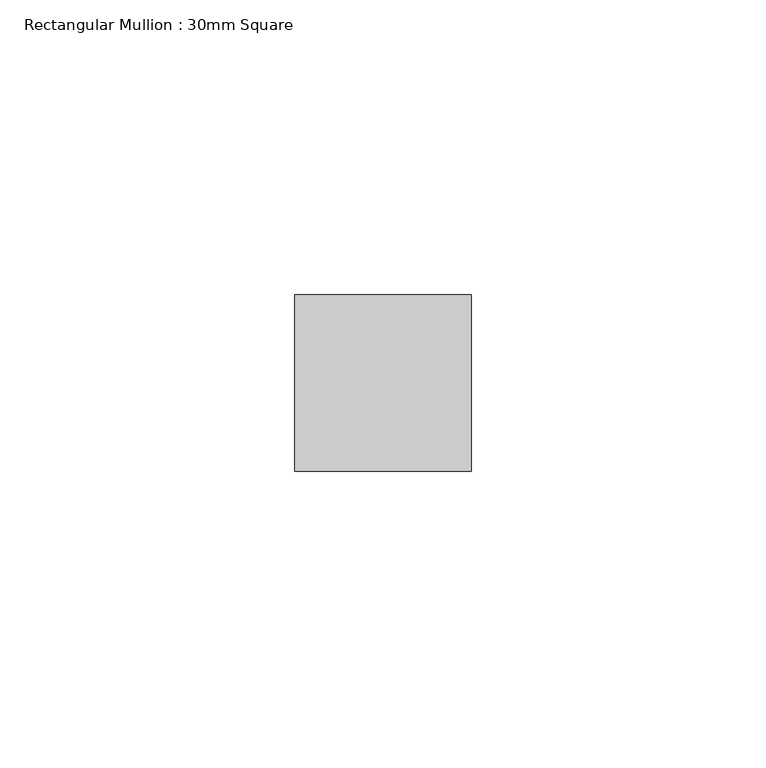
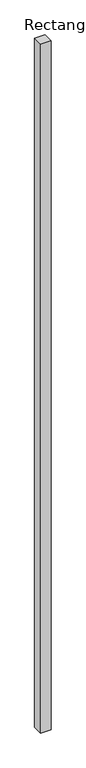
"""IFC4 building model written with IfcOpenShell, lengths in millimetres: member geometry, Rectangular Mullion : 30mm Square."""

import ifcopenshell
import ifcopenshell.guid

model = None  # the IFC model being written
_history = None  # IfcOwnerHistory: only IFC2X3 demands one
_inside = {}  # id of a spatial element -> (the spatial element, [elements in it])
_under = {}  # id of a project, library or spatial element -> (it, [spatial elements below it])
_declared = {}  # id of a project -> (the project, [libraries it declares])
_typed = {}  # id of a type object -> (the type object, [elements of that type])
_made_of = {}  # id of a material, layer set ... -> (it, [elements and type objects made of it])


def new_model(schema):
    """Start an empty IFC model of exactly this schema.

    Asked for "IFC4X3", IfcOpenShell would pick the latest addendum, in which some entities
    have other attributes; the version numbers below select the first issue.
    IFC2X3 requires an IfcOwnerHistory on every rooted entity: one is made here for all.
    """
    global model, _history
    if schema == "IFC4X3":
        model = ifcopenshell.file(schema_version=(4, 3, 0, 0))
    else:
        model = ifcopenshell.file(schema=schema)
    _inside.clear()
    _under.clear()
    _declared.clear()
    _typed.clear()
    _made_of.clear()
    _history = None
    if model.schema == "IFC2X3":
        org = make("IfcOrganization", Name="unknown")
        user = make(
            "IfcPersonAndOrganization",
            ThePerson=make("IfcPerson", FamilyName="unknown"),
            TheOrganization=org,
        )
        app = make(
            "IfcApplication",
            ApplicationDeveloper=org,
            Version="unknown",
            ApplicationFullName="unknown",
            ApplicationIdentifier="unknown",
        )
        _history = make(
            "IfcOwnerHistory",
            OwningUser=user,
            OwningApplication=app,
            ChangeAction="ADDED",
            CreationDate=0,
        )
    return model


def make(cls, **values):
    """One entity of the class cls with the attributes given. An attribute that is None is left unset."""
    return model.create_entity(
        cls, **{name: value for name, value in values.items() if value is not None}
    )


def rooted(cls, **values):
    """An entity with a GlobalId (a new one), such as an element, a storey or a relation."""
    return make(cls, GlobalId=ifcopenshell.guid.new(), OwnerHistory=_history, **values)


def si_unit(unit_type, name, prefix=None):
    """IfcSIUnit, for example si_unit("LENGTHUNIT", "METRE", prefix="MILLI")."""
    return make("IfcSIUnit", UnitType=unit_type, Prefix=prefix, Name=name)


def assignment(units):
    """IfcUnitAssignment: the units of a project."""
    return None if units is None else make("IfcUnitAssignment", Units=units)


def point(xyz):
    """IfcCartesianPoint."""
    return None if xyz is None else make("IfcCartesianPoint", Coordinates=xyz)


def direction(xyz):
    """IfcDirection."""
    return None if xyz is None else make("IfcDirection", DirectionRatios=xyz)


def frame(location, z_axis=None, x_axis=None):
    """IfcAxis2Placement3D, a coordinate frame: its origin and axes. An axis left out is left unset."""
    return make(
        "IfcAxis2Placement3D",
        Location=point(location),
        Axis=direction(z_axis),
        RefDirection=direction(x_axis),
    )


def origin():
    """The frame at (0, 0, 0) with its axes left unset."""
    return frame((0.0, 0.0, 0.0))


def place(relative_to, where):
    """IfcLocalPlacement: puts the frame where relative to a parent placement (None: the world)."""
    return make(
        "IfcLocalPlacement", PlacementRelTo=relative_to, RelativePlacement=where
    )


def context(
    kind, dimensions, precision=None, world=None, true_north=None, identifier=None
):
    """IfcGeometricRepresentationContext, for example the 3D "Model" context."""
    return make(
        "IfcGeometricRepresentationContext",
        ContextIdentifier=identifier,
        ContextType=kind,
        CoordinateSpaceDimension=dimensions,
        Precision=precision,
        WorldCoordinateSystem=world,
        TrueNorth=true_north,
    )


def project(units=None, contexts=None):
    """IfcProject with its units and contexts."""
    return rooted(
        "IfcProject",
        Name="project",
        RepresentationContexts=contexts,
        UnitsInContext=assignment(units),
    )


def spatial(cls, under=None, at=None, **own):
    """A site, building, storey or space (cls), placed at a placement, below another one or the project."""
    s = rooted(cls, ObjectPlacement=at, **own)
    if under is not None:
        _under.setdefault(under.id(), (under, []))[1].append(s)
    return s


def polyline(points):
    """IfcPolyline through the points."""
    return make("IfcPolyline", Points=[point(p) for p in points])


def outline(outer, holes=None, kind="AREA"):
    """IfcArbitraryClosedProfileDef: a profile drawn as a closed curve; with holes, ...WithVoids."""
    if holes is None:
        return make("IfcArbitraryClosedProfileDef", ProfileType=kind, OuterCurve=outer)
    return make(
        "IfcArbitraryProfileDefWithVoids",
        ProfileType=kind,
        OuterCurve=outer,
        InnerCurves=holes,
    )


def extrude(swept, where, along, depth):
    """IfcExtrudedAreaSolid: the profile swept, set in the frame where, extruded along a direction by depth."""
    return make(
        "IfcExtrudedAreaSolid",
        SweptArea=swept,
        Position=where,
        ExtrudedDirection=direction(along),
        Depth=depth,
    )


def shape(context_of_items, identifier, shape_type, items):
    """IfcShapeRepresentation: the items that make up one representation, for example the "Body"."""
    return make(
        "IfcShapeRepresentation",
        ContextOfItems=context_of_items,
        RepresentationIdentifier=identifier,
        RepresentationType=shape_type,
        Items=items,
    )


def source(mapping_origin, context_of_items, identifier, shape_type, items):
    """IfcRepresentationMap: a shape defined once, which mapped items show again and again."""
    return make(
        "IfcRepresentationMap",
        MappingOrigin=mapping_origin,
        MappedRepresentation=shape(context_of_items, identifier, shape_type, items),
    )


def transform(
    local_origin,
    x_axis=None,
    y_axis=None,
    z_axis=None,
    scale=None,
    scale2=None,
    scale3=None,
    uniform=True,
):
    """IfcCartesianTransformationOperator3D, or its non-uniform kind. x_axis, y_axis, z_axis: its Axis1, 2, 3."""
    if uniform:
        return make(
            "IfcCartesianTransformationOperator3D",
            Axis1=direction(x_axis),
            Axis2=direction(y_axis),
            LocalOrigin=point(local_origin),
            Scale=scale,
            Axis3=direction(z_axis),
        )
    return make(
        "IfcCartesianTransformationOperator3DnonUniform",
        Axis1=direction(x_axis),
        Axis2=direction(y_axis),
        LocalOrigin=point(local_origin),
        Scale=scale,
        Axis3=direction(z_axis),
        Scale2=scale2,
        Scale3=scale3,
    )


def mapped(mapping_source, mapping_target):
    """IfcMappedItem: shows the shape of a source again, moved by a transform."""
    return make(
        "IfcMappedItem", MappingSource=mapping_source, MappingTarget=mapping_target
    )


def made_of(thing, what):
    """Note that an element or type object is made of a material, layer set ...; save() writes the relation."""
    if what is not None:
        _made_of.setdefault(what.id(), (what, []))[1].append(thing)
    return thing


def element(
    cls,
    number,
    at=None,
    inside=None,
    cuts=None,
    type_object=None,
    material=None,
    context=None,
    identifier="Body",
    shape_type=None,
    held_by="IfcProductDefinitionShape",
    body=None,
    shapes=None,
    **own,
):
    """One element of the class cls, such as IfcWall. Its Tag is "e" and its number.

    at: its placement. inside: the storey or other place that contains it. cuts: it is an
    opening in that element (IfcRelVoidsElement). A single representation is given by context,
    identifier, shape_type and body (its items); several are given by shapes. held_by: the class
    of the entity that holds the representations. save() writes the other relations.
    """
    e = rooted(cls, Tag="e%d" % number, ObjectPlacement=at, **own)
    if body is not None:
        shapes = [shape(context, identifier, shape_type, body)]
    if shapes is not None:
        e.Representation = make(held_by, Representations=shapes)
    if inside is not None:
        _inside.setdefault(inside.id(), (inside, []))[1].append(e)
    if cuts is not None:
        rooted(
            "IfcRelVoidsElement", RelatingBuildingElement=cuts, RelatedOpeningElement=e
        )
    if type_object is not None:
        _typed.setdefault(type_object.id(), (type_object, []))[1].append(e)
    return made_of(e, material)


def aggregate(whole, parts):
    """IfcRelAggregates: a whole, such as a stair, and the parts it consists of."""
    return rooted("IfcRelAggregates", RelatingObject=whole, RelatedObjects=parts)


def save(model, path):
    """Write the relations noted so far, then the file.

    IfcRelAggregates (storeys below a building ...), IfcRelContainedInSpatialStructure (elements
    in a storey), IfcRelDefinesByType, IfcRelAssociatesMaterial and IfcRelDeclares: one each for
    every whole, place, type object, material and project.
    """
    for whole, parts in _under.values():
        aggregate(whole, parts)
    for where, things in _inside.values():
        rooted(
            "IfcRelContainedInSpatialStructure",
            RelatedElements=things,
            RelatingStructure=where,
        )
    for kind, things in _typed.values():
        rooted("IfcRelDefinesByType", RelatedObjects=things, RelatingType=kind)
    for what, things in _made_of.values():
        rooted("IfcRelAssociatesMaterial", RelatedObjects=things, RelatingMaterial=what)
    for by, libraries in _declared.values():
        rooted("IfcRelDeclares", RelatingContext=by, RelatedDefinitions=libraries)
    model.write(path)


def rectangular_mullion_30mm_square_12e3d361(model_context):
    return source(origin(), model_context, "Body", "SweptSolid", [
        extrude(outline(polyline([(15.0, 15.0), (15.0, -15.0), (-15.0, -15.0), (-15.0, 15.0), (15.0, 15.0)])), frame((0.0, 0.0, -2100.6682892), z_axis=(0.0, 0.0, 1.0), x_axis=(1.0, 0.0, 0.0)), (0.0, 0.0, 1.0), 2100.6682892),
    ])


if __name__ == "__main__":
    model = new_model("IFC4")
    model_context = context("Model", 3, world=origin())
    ifc_project = project(units=[si_unit("LENGTHUNIT", "METRE", prefix="MILLI")], contexts=[model_context])
    site = spatial("IfcSite", under=ifc_project)
    building = spatial("IfcBuilding", under=site)
    placement = place(None, origin())
    rectangular_mullion_30mm_square_shape = rectangular_mullion_30mm_square_12e3d361(model_context)
    element("IfcMember", 1, ObjectType="Rectangular Mullion : 30mm Square", at=placement, inside=building, context=model_context, shape_type="MappedRepresentation", body=[
        mapped(rectangular_mullion_30mm_square_shape, transform((0.0, 0.0, 0.0), x_axis=(1.0, 0.0, 0.0), y_axis=(0.0, 1.0, 0.0), z_axis=(0.0, 0.0, 1.0))),
    ])
    save(model, "model.ifc")

# Revit data of these elements
# Type "Rectangular Mullion : 30mm Square"
#   built-in parameter 1007304 = 0.0984252 (stored number, unit not read)
#   built-in parameter 1007301 = 0.0492126 (stored number, unit not read)
#   built-in parameter 1007300 = 0.0492126 (stored number, unit not read)
# Element 1 (IfcMember, "Rectangular Mullion : 30mm Square")
#   Materials on its faces: "Aluminum"
# Materials
#   "Aluminum": class "Metal", colour RGB 244 244 244, transparency 0, Description = "Aluminum 6061", Cost = 0
